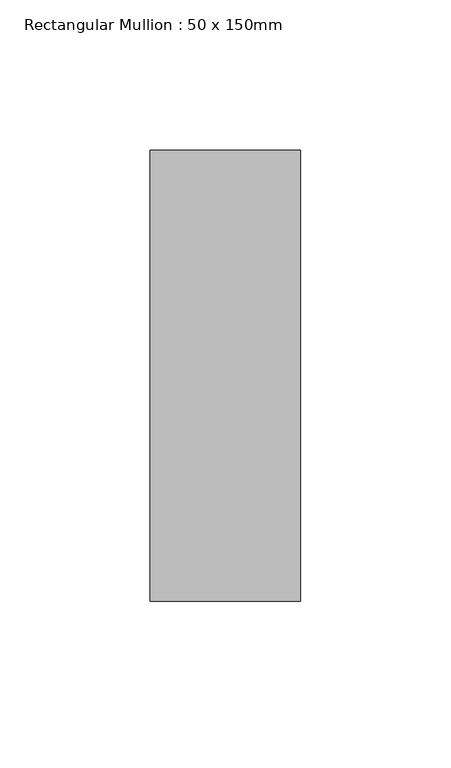
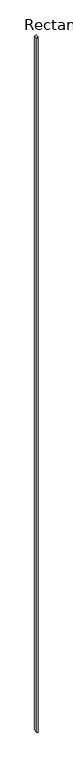
"""IFC4 building model written with IfcOpenShell, lengths in millimetres: member geometry, Rectangular Mullion : 50 x 150mm."""

import ifcopenshell
import ifcopenshell.guid

model = None  # the IFC model being written
_history = None  # IfcOwnerHistory: only IFC2X3 demands one
_inside = {}  # id of a spatial element -> (the spatial element, [elements in it])
_under = {}  # id of a project, library or spatial element -> (it, [spatial elements below it])
_declared = {}  # id of a project -> (the project, [libraries it declares])
_typed = {}  # id of a type object -> (the type object, [elements of that type])
_made_of = {}  # id of a material, layer set ... -> (it, [elements and type objects made of it])


def new_model(schema):
    """Start an empty IFC model of exactly this schema.

    Asked for "IFC4X3", IfcOpenShell would pick the latest addendum, in which some entities
    have other attributes; the version numbers below select the first issue.
    IFC2X3 requires an IfcOwnerHistory on every rooted entity: one is made here for all.
    """
    global model, _history
    if schema == "IFC4X3":
        model = ifcopenshell.file(schema_version=(4, 3, 0, 0))
    else:
        model = ifcopenshell.file(schema=schema)
    _inside.clear()
    _under.clear()
    _declared.clear()
    _typed.clear()
    _made_of.clear()
    _history = None
    if model.schema == "IFC2X3":
        org = make("IfcOrganization", Name="unknown")
        user = make(
            "IfcPersonAndOrganization",
            ThePerson=make("IfcPerson", FamilyName="unknown"),
            TheOrganization=org,
        )
        app = make(
            "IfcApplication",
            ApplicationDeveloper=org,
            Version="unknown",
            ApplicationFullName="unknown",
            ApplicationIdentifier="unknown",
        )
        _history = make(
            "IfcOwnerHistory",
            OwningUser=user,
            OwningApplication=app,
            ChangeAction="ADDED",
            CreationDate=0,
        )
    return model


def make(cls, **values):
    """One entity of the class cls with the attributes given. An attribute that is None is left unset."""
    return model.create_entity(
        cls, **{name: value for name, value in values.items() if value is not None}
    )


def rooted(cls, **values):
    """An entity with a GlobalId (a new one), such as an element, a storey or a relation."""
    return make(cls, GlobalId=ifcopenshell.guid.new(), OwnerHistory=_history, **values)


def si_unit(unit_type, name, prefix=None):
    """IfcSIUnit, for example si_unit("LENGTHUNIT", "METRE", prefix="MILLI")."""
    return make("IfcSIUnit", UnitType=unit_type, Prefix=prefix, Name=name)


def assignment(units):
    """IfcUnitAssignment: the units of a project."""
    return None if units is None else make("IfcUnitAssignment", Units=units)


def point(xyz):
    """IfcCartesianPoint."""
    return None if xyz is None else make("IfcCartesianPoint", Coordinates=xyz)


def direction(xyz):
    """IfcDirection."""
    return None if xyz is None else make("IfcDirection", DirectionRatios=xyz)


def frame(location, z_axis=None, x_axis=None):
    """IfcAxis2Placement3D, a coordinate frame: its origin and axes. An axis left out is left unset."""
    return make(
        "IfcAxis2Placement3D",
        Location=point(location),
        Axis=direction(z_axis),
        RefDirection=direction(x_axis),
    )


def origin():
    """The frame at (0, 0, 0) with its axes left unset."""
    return frame((0.0, 0.0, 0.0))


def place(relative_to, where):
    """IfcLocalPlacement: puts the frame where relative to a parent placement (None: the world)."""
    return make(
        "IfcLocalPlacement", PlacementRelTo=relative_to, RelativePlacement=where
    )


def context(
    kind, dimensions, precision=None, world=None, true_north=None, identifier=None
):
    """IfcGeometricRepresentationContext, for example the 3D "Model" context."""
    return make(
        "IfcGeometricRepresentationContext",
        ContextIdentifier=identifier,
        ContextType=kind,
        CoordinateSpaceDimension=dimensions,
        Precision=precision,
        WorldCoordinateSystem=world,
        TrueNorth=true_north,
    )


def project(units=None, contexts=None):
    """IfcProject with its units and contexts."""
    return rooted(
        "IfcProject",
        Name="project",
        RepresentationContexts=contexts,
        UnitsInContext=assignment(units),
    )


def spatial(cls, under=None, at=None, **own):
    """A site, building, storey or space (cls), placed at a placement, below another one or the project."""
    s = rooted(cls, ObjectPlacement=at, **own)
    if under is not None:
        _under.setdefault(under.id(), (under, []))[1].append(s)
    return s


def polyline(points):
    """IfcPolyline through the points."""
    return make("IfcPolyline", Points=[point(p) for p in points])


def outline(outer, holes=None, kind="AREA"):
    """IfcArbitraryClosedProfileDef: a profile drawn as a closed curve; with holes, ...WithVoids."""
    if holes is None:
        return make("IfcArbitraryClosedProfileDef", ProfileType=kind, OuterCurve=outer)
    return make(
        "IfcArbitraryProfileDefWithVoids",
        ProfileType=kind,
        OuterCurve=outer,
        InnerCurves=holes,
    )


def extrude(swept, where, along, depth):
    """IfcExtrudedAreaSolid: the profile swept, set in the frame where, extruded along a direction by depth."""
    return make(
        "IfcExtrudedAreaSolid",
        SweptArea=swept,
        Position=where,
        ExtrudedDirection=direction(along),
        Depth=depth,
    )


def shape(context_of_items, identifier, shape_type, items):
    """IfcShapeRepresentation: the items that make up one representation, for example the "Body"."""
    return make(
        "IfcShapeRepresentation",
        ContextOfItems=context_of_items,
        RepresentationIdentifier=identifier,
        RepresentationType=shape_type,
        Items=items,
    )


def source(mapping_origin, context_of_items, identifier, shape_type, items):
    """IfcRepresentationMap: a shape defined once, which mapped items show again and again."""
    return make(
        "IfcRepresentationMap",
        MappingOrigin=mapping_origin,
        MappedRepresentation=shape(context_of_items, identifier, shape_type, items),
    )


def transform(
    local_origin,
    x_axis=None,
    y_axis=None,
    z_axis=None,
    scale=None,
    scale2=None,
    scale3=None,
    uniform=True,
):
    """IfcCartesianTransformationOperator3D, or its non-uniform kind. x_axis, y_axis, z_axis: its Axis1, 2, 3."""
    if uniform:
        return make(
            "IfcCartesianTransformationOperator3D",
            Axis1=direction(x_axis),
            Axis2=direction(y_axis),
            LocalOrigin=point(local_origin),
            Scale=scale,
            Axis3=direction(z_axis),
        )
    return make(
        "IfcCartesianTransformationOperator3DnonUniform",
        Axis1=direction(x_axis),
        Axis2=direction(y_axis),
        LocalOrigin=point(local_origin),
        Scale=scale,
        Axis3=direction(z_axis),
        Scale2=scale2,
        Scale3=scale3,
    )


def mapped(mapping_source, mapping_target):
    """IfcMappedItem: shows the shape of a source again, moved by a transform."""
    return make(
        "IfcMappedItem", MappingSource=mapping_source, MappingTarget=mapping_target
    )


def made_of(thing, what):
    """Note that an element or type object is made of a material, layer set ...; save() writes the relation."""
    if what is not None:
        _made_of.setdefault(what.id(), (what, []))[1].append(thing)
    return thing


def element(
    cls,
    number,
    at=None,
    inside=None,
    cuts=None,
    type_object=None,
    material=None,
    context=None,
    identifier="Body",
    shape_type=None,
    held_by="IfcProductDefinitionShape",
    body=None,
    shapes=None,
    **own,
):
    """One element of the class cls, such as IfcWall. Its Tag is "e" and its number.

    at: its placement. inside: the storey or other place that contains it. cuts: it is an
    opening in that element (IfcRelVoidsElement). A single representation is given by context,
    identifier, shape_type and body (its items); several are given by shapes. held_by: the class
    of the entity that holds the representations. save() writes the other relations.
    """
    e = rooted(cls, Tag="e%d" % number, ObjectPlacement=at, **own)
    if body is not None:
        shapes = [shape(context, identifier, shape_type, body)]
    if shapes is not None:
        e.Representation = make(held_by, Representations=shapes)
    if inside is not None:
        _inside.setdefault(inside.id(), (inside, []))[1].append(e)
    if cuts is not None:
        rooted(
            "IfcRelVoidsElement", RelatingBuildingElement=cuts, RelatedOpeningElement=e
        )
    if type_object is not None:
        _typed.setdefault(type_object.id(), (type_object, []))[1].append(e)
    return made_of(e, material)


def aggregate(whole, parts):
    """IfcRelAggregates: a whole, such as a stair, and the parts it consists of."""
    return rooted("IfcRelAggregates", RelatingObject=whole, RelatedObjects=parts)


def save(model, path):
    """Write the relations noted so far, then the file.

    IfcRelAggregates (storeys below a building ...), IfcRelContainedInSpatialStructure (elements
    in a storey), IfcRelDefinesByType, IfcRelAssociatesMaterial and IfcRelDeclares: one each for
    every whole, place, type object, material and project.
    """
    for whole, parts in _under.values():
        aggregate(whole, parts)
    for where, things in _inside.values():
        rooted(
            "IfcRelContainedInSpatialStructure",
            RelatedElements=things,
            RelatingStructure=where,
        )
    for kind, things in _typed.values():
        rooted("IfcRelDefinesByType", RelatedObjects=things, RelatingType=kind)
    for what, things in _made_of.values():
        rooted("IfcRelAssociatesMaterial", RelatedObjects=things, RelatingMaterial=what)
    for by, libraries in _declared.values():
        rooted("IfcRelDeclares", RelatingContext=by, RelatedDefinitions=libraries)
    model.write(path)


def rectangular_mullion_50_x_150mm_0c0d54b6(model_context):
    return source(origin(), model_context, "Body", "SweptSolid", [
        extrude(outline(polyline([(0.0, 0.0), (-53.1084457, -50.0), (-31009.3272322, -50.0), (-31056.4007243, 0.0), (0.0, 0.0)])), frame((0.0, -75.0, 0.0), z_axis=(0.0, 1.0, 0.0), x_axis=(0.0, 0.0, 1.0)), (0.0, 0.0, 1.0), 150.0),
    ])


if __name__ == "__main__":
    model = new_model("IFC4")
    model_context = context("Model", 3, world=origin())
    ifc_project = project(units=[si_unit("LENGTHUNIT", "METRE", prefix="MILLI")], contexts=[model_context])
    site = spatial("IfcSite", under=ifc_project)
    building = spatial("IfcBuilding", under=site)
    placement = place(None, origin())
    rectangular_mullion_50_x_150mm_shape = rectangular_mullion_50_x_150mm_0c0d54b6(model_context)
    element("IfcMember", 1, ObjectType="Rectangular Mullion : 50 x 150mm", at=placement, inside=building, context=model_context, shape_type="MappedRepresentation", body=[
        mapped(rectangular_mullion_50_x_150mm_shape, transform((0.0, 0.0, 0.0), x_axis=(1.0, 0.0, 0.0), y_axis=(0.0, 1.0, 0.0), z_axis=(0.0, 0.0, 1.0))),
    ])
    save(model, "model.ifc")

# Revit data of these elements
# Type "Rectangular Mullion : 50 x 150mm"
#   built-in parameter 1007304 = 0.492126 (stored number, unit not read)
#   built-in parameter 1007301 = 0.082021 (stored number, unit not read)
#   built-in parameter 1007300 = 0.082021 (stored number, unit not read)
# Element 1 (IfcMember, "Rectangular Mullion : 50 x 150mm")
#   Materials on its faces: "Metal - Aluminium"
# Materials
#   "Metal - Aluminium": class "Metal", colour RGB 247 247 247, transparency 0
